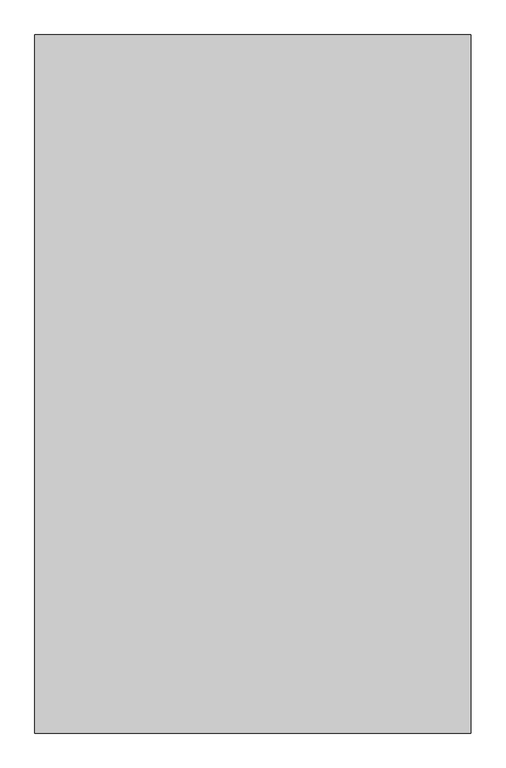
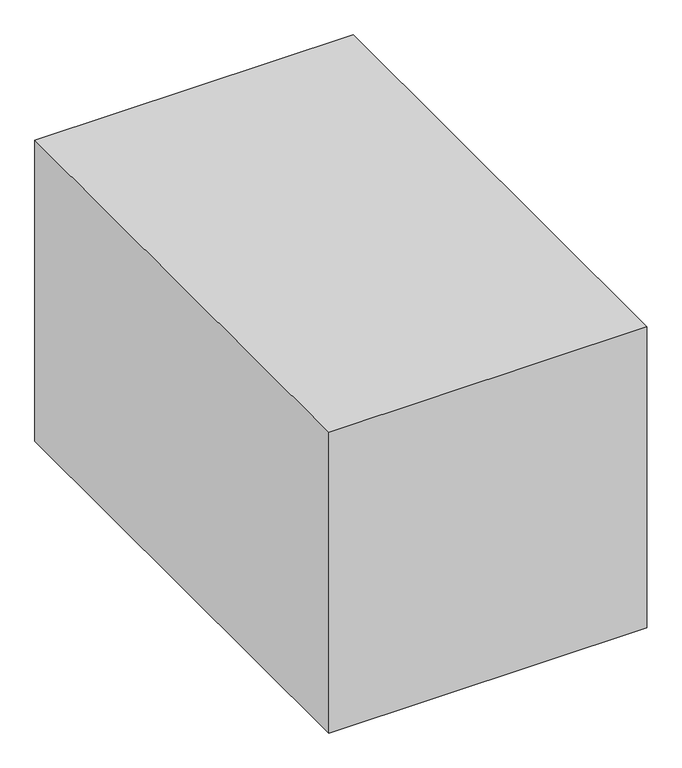
"""IFC4 building model written with IfcOpenShell, lengths in millimetres: proxy geometry, Space Planning Box_hec : Space Planning Box_hec."""

from ifc_helpers import new_model, si_unit, origin, origin_with_axes, place, context, project, spatial, polyline, outline, extrude, source, transform, mapped, element, save


def generic_models_b37916ea(model_context):
    return source(origin(), model_context, "Body", "SweptSolid", [
        extrude(outline(polyline([(1750.0, 2800.0), (1750.0, -2800.0), (-1750.0, -2800.0), (-1750.0, 2800.0), (1750.0, 2800.0)])), origin_with_axes(), (0.0, 0.0, 1.0), 3500.0),
    ])


if __name__ == "__main__":
    model = new_model("IFC4")
    model_context = context("Model", 3, world=origin())
    ifc_project = project(units=[si_unit("LENGTHUNIT", "METRE", prefix="MILLI")], contexts=[model_context])
    site = spatial("IfcSite", under=ifc_project)
    building = spatial("IfcBuilding", under=site)
    placement = place(None, origin())
    generic_models_shape = generic_models_b37916ea(model_context)
    element("IfcBuildingElementProxy", 1, Name="Space Planning Box_hec : Space Planning Box_hec", ObjectType="Space Planning Box_hec : Space Planning Box_hec", at=placement, inside=building, context=model_context, shape_type="MappedRepresentation", body=[
        mapped(generic_models_shape, transform((0.0, 0.0, 0.0), x_axis=(1.0, 0.0, 0.0), y_axis=(0.0, 1.0, 0.0), z_axis=(0.0, 0.0, 1.0))),
    ])
    save(model, "model.ifc")

# Revit data of these elements
# Type "Space Planning Box_hec : Space Planning Box_hec"
#   Type Comments = "..."
#   Room Name [instance default] = "?"
#   Interior Finish [instance default] = ""
#   Exterior Finish [instance default] = ""
#   Department [instance default] = ""
#   Assembly Code = "..."
#   ceiling height [instance default] = 0
#   Width [instance default] = 1524 mm
#   Program Area [instance default] = 0.00 m²
#   Length [instance default] = 1524 mm
#   Height [instance default] = 1524 mm
#   Area [instance default] = 2.32258 m²
#   Fill Color [instance default] = Cyan
#   Default Elevation = 0
# Element 1 (IfcBuildingElementProxy, "Space Planning Box_hec : Space Planning Box_hec")
#   Room Name = "Toilet"
#   Exterior Finish = "RF1..N/A,,N/A..N/A..N/A"
#   Department = "AR"
#   Width = 3500 mm
#   Program Area = 19.60 m²
#   Length = 5600 mm
#   Height = 3500 mm
#   Area = 19.60 m²
#   Materials on its faces: "Cyan"
# Materials
#   "Cyan": class "Generic", colour RGB 0 255 255, transparency 0.2, Cost = 0
